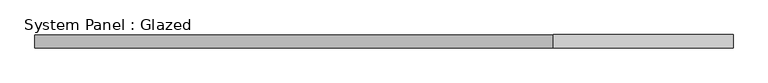
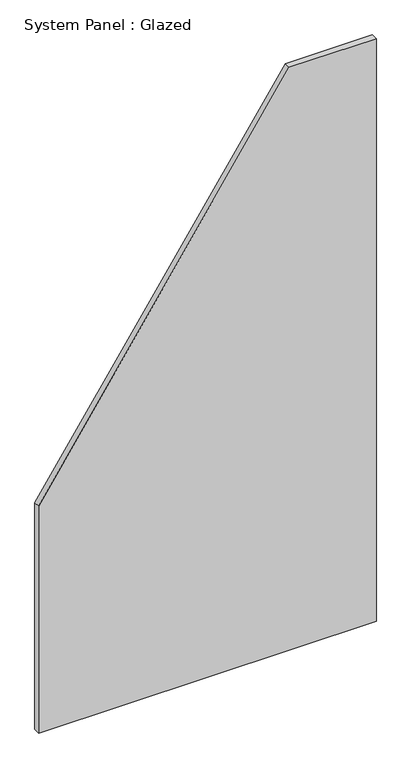
"""IFC4 building model written with IfcOpenShell, lengths in millimetres: plate geometry, System Panel : Glazed."""

from ifc_helpers import new_model, si_unit, frame, origin, place, context, project, spatial, polyline, outline, extrude, source, transform, mapped, element, save


def system_panel_glazed_2a40db34(model_context):
    return source(origin(), model_context, "Body", "SweptSolid", [
        extrude(outline(polyline([(0.0, -658.3333333), (0.0, 658.3333333), (2400.0, 658.3333333), (2400.0, 318.9382443), (934.2941385, -658.3333333), (0.0, -658.3333333)])), frame((0.0, 24.5, 0.0), z_axis=(0.0, 1.0, 0.0), x_axis=(0.0, 0.0, 1.0)), (0.0, 0.0, 1.0), 25.0),
    ])


if __name__ == "__main__":
    model = new_model("IFC4")
    model_context = context("Model", 3, world=origin())
    ifc_project = project(units=[si_unit("LENGTHUNIT", "METRE", prefix="MILLI")], contexts=[model_context])
    site = spatial("IfcSite", under=ifc_project)
    building = spatial("IfcBuilding", under=site)
    placement = place(None, origin())
    system_panel_glazed_shape = system_panel_glazed_2a40db34(model_context)
    element("IfcPlate", 1, ObjectType="System Panel : Glazed", at=placement, inside=building, context=model_context, shape_type="MappedRepresentation", body=[
        mapped(system_panel_glazed_shape, transform((0.0, 0.0, 0.0), x_axis=(1.0, 0.0, 0.0), y_axis=(0.0, 1.0, 0.0), z_axis=(0.0, 0.0, 1.0))),
    ])
    save(model, "model.ifc")

# Revit data of these elements
# Type "System Panel : Glazed"
#   Keynote = "H11"
#   Construction Type Id = "GSP4R"
#   Analytic Construction = "1/8 in Pilkington single glazing"
#   Visual Light Transmittance = 0.9
#   Solar Heat Gain Coefficient = 0.86
#   Heat Transfer Coefficient (U) = 6.7069 W/(m²·K)
#   Define Thermal Properties by = 1
# Element 1 (IfcPlate, "System Panel : Glazed")
#   Materials on its faces: "Glass"
# Materials
#   "Glass": class "Glass", colour RGB 0 128 192, transparency 0.9, Description = "Soda Lime Glass", Cost = 0
